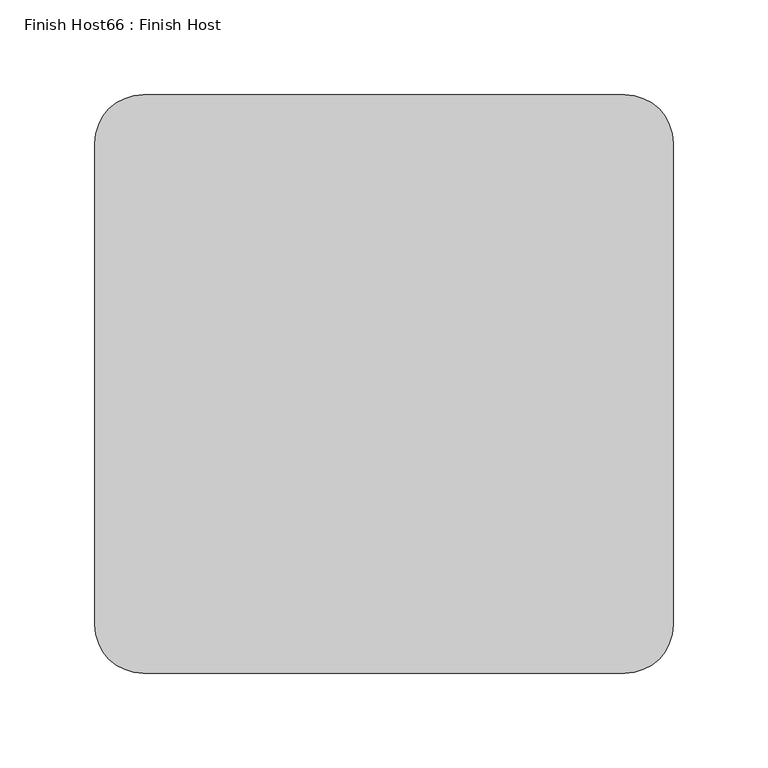
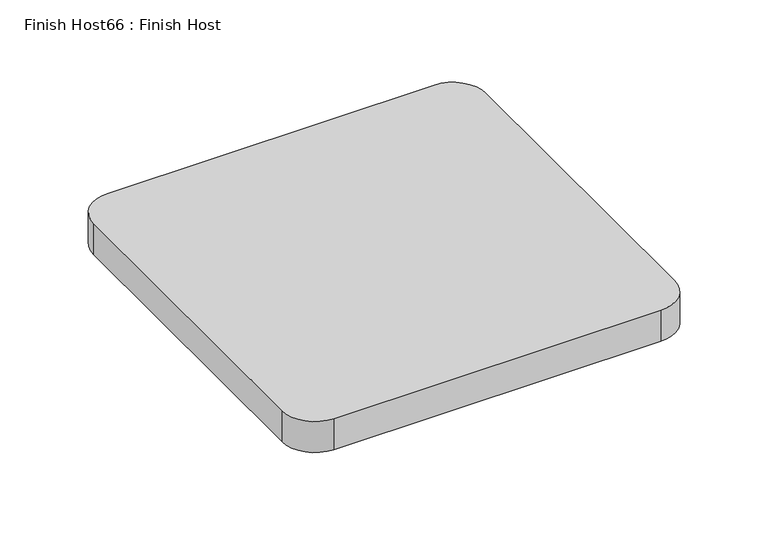
"""IFC4 building model written with IfcOpenShell, lengths in millimetres: proxy geometry, Finish Host66 : Finish Host."""

from ifc_helpers import new_model, si_unit, point, frame_2d, origin, origin_with_axes, place, context, project, spatial, polyline, circle_curve, trimmed, segment, composite_curve, outline, extrude, source, transform, mapped, element, save


def finish_host66_finish_host_af9bd7ae(model_context):
    return source(origin(), model_context, "Body", "SweptSolid", [
        extrude(outline(composite_curve([segment(polyline([(-11384.2801686, 10745.5913835), (-11384.2801686, 10999.5913835)]), True, "CONTINUOUS"), segment(trimmed(circle_curve(frame_2d((-11358.8801686, 10999.5913835)), 25.4), [point((-11384.2801686, 10999.5913835))], [point((-11358.8801686, 11024.9913835))], False, "CARTESIAN"), True, "CONTINUOUS"), segment(polyline([(-11358.8801686, 11024.9913835), (-11104.8801686, 11024.9913835)]), True, "CONTINUOUS"), segment(trimmed(circle_curve(frame_2d((-11104.8801686, 10999.5913835)), 25.4), [point((-11104.8801686, 11024.9913835))], [point((-11079.4801686, 10999.5913835))], False, "CARTESIAN"), True, "CONTINUOUS"), segment(polyline([(-11079.4801686, 10999.5913835), (-11079.4801686, 10745.5913835)]), True, "CONTINUOUS"), segment(trimmed(circle_curve(frame_2d((-11104.8801686, 10745.5913835)), 25.4), [point((-11079.4801686, 10745.5913835))], [point((-11104.8801686, 10720.1913835))], False, "CARTESIAN"), True, "CONTINUOUS"), segment(polyline([(-11104.8801686, 10720.1913835), (-11358.8801686, 10720.1913835)]), True, "CONTINUOUS"), segment(trimmed(circle_curve(frame_2d((-11358.8801686, 10745.5913835)), 25.4), [point((-11358.8801686, 10720.1913835))], [point((-11384.2801686, 10745.5913835))], False, "CARTESIAN"), True, "CONTINUOUS")], self_intersect=False)), origin_with_axes(), (0.0, 0.0, 1.0), 25.4),
    ])


if __name__ == "__main__":
    model = new_model("IFC4")
    model_context = context("Model", 3, world=origin())
    ifc_project = project(units=[si_unit("LENGTHUNIT", "METRE", prefix="MILLI")], contexts=[model_context])
    site = spatial("IfcSite", under=ifc_project)
    building = spatial("IfcBuilding", under=site)
    placement = place(None, origin())
    finish_host66_finish_host_shape = finish_host66_finish_host_af9bd7ae(model_context)
    element("IfcBuildingElementProxy", 1, Name="Finish Host66 : Finish Host", ObjectType="Finish Host66 : Finish Host", at=placement, inside=building, context=model_context, shape_type="MappedRepresentation", body=[
        mapped(finish_host66_finish_host_shape, transform((0.0, 0.0, 0.0), x_axis=(1.0, 0.0, 0.0), y_axis=(0.0, 1.0, 0.0), z_axis=(0.0, 0.0, 1.0))),
    ])
    save(model, "model.ifc")

# Revit data of these elements
# Type "Finish Host66 : Finish Host"
#   Countertop Material = Wood - Teknion - MP - Natural Maple
# Element 1 (IfcBuildingElementProxy, "Finish Host66 : Finish Host")
#   Materials on its faces: "Wood - Teknion - MP - Natural Maple"
# Materials
#   "Wood - Teknion - MP - Natural Maple": class "Wood", colour RGB 128 121 105, transparency 0, Model = "MP", Manufacturer = "Teknion Studio", URL = "http://www.teknion.com/", Description = "Natural Maple", Cost = 0
